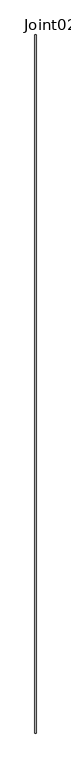
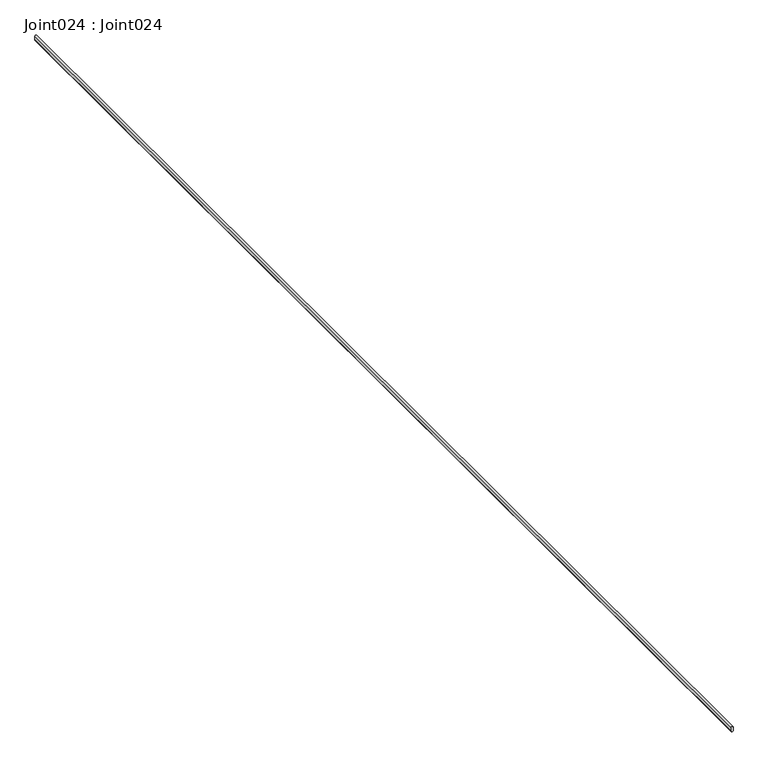
"""IFC4 building model written with IfcOpenShell, lengths in millimetres: proxy geometry, Joint024 : Joint024."""

from ifc_helpers import new_model, si_unit, point, frame, frame_2d, origin, place, context, project, spatial, polyline, circle_curve, trimmed, segment, composite_curve, outline, extrude, source, transform, mapped, element, save


def joint024_joint024_37bc9509(model_context):
    return source(origin(), model_context, "Body", "SweptSolid", [
        extrude(outline(composite_curve([segment(polyline([(42015.0117187, -1061.5223389), (42020.9666748, -1061.5223389)]), True, "CONTINUOUS"), segment(trimmed(circle_curve(frame_2d((42020.9666748, -1063.1082764)), 1.5859375), [point((42020.9666748, -1061.5223389))], [point((42020.9666748, -1064.6942139))], False, "CARTESIAN"), True, "CONTINUOUS"), segment(polyline([(42020.9666748, -1064.6942139), (42015.0117187, -1064.6942139)]), True, "CONTINUOUS"), segment(trimmed(circle_curve(frame_2d((42015.0117187, -1063.1082764)), 1.5859375), [point((42015.0117187, -1064.6942139))], [point((42015.0117187, -1061.5223389))], False, "CARTESIAN"), True, "CONTINUOUS")], self_intersect=False)), frame((0.0, -1052.8906544, 0.0), z_axis=(0.0, 1.0, 0.0), x_axis=(0.0, 0.0, 1.0)), (0.0, 0.0, 1.0), 2000.0),
    ])


if __name__ == "__main__":
    model = new_model("IFC4")
    model_context = context("Model", 3, world=origin())
    ifc_project = project(units=[si_unit("LENGTHUNIT", "METRE", prefix="MILLI")], contexts=[model_context])
    site = spatial("IfcSite", under=ifc_project)
    building = spatial("IfcBuilding", under=site)
    placement = place(None, origin())
    joint024_joint024_shape = joint024_joint024_37bc9509(model_context)
    element("IfcBuildingElementProxy", 1, Name="Joint024 : Joint024", ObjectType="Joint024 : Joint024", at=placement, inside=building, context=model_context, shape_type="MappedRepresentation", body=[
        mapped(joint024_joint024_shape, transform((0.0, 0.0, 0.0), x_axis=(1.0, 0.0, 0.0), y_axis=(0.0, 1.0, 0.0), z_axis=(0.0, 0.0, 1.0))),
    ])
    save(model, "model.ifc")

# Revit data of these elements
# Type "Joint024 : Joint024"
#   NameOverride = "Joint024"
# Element 1 (IfcBuildingElementProxy, "Joint024 : Joint024")
#   Materials on its faces: "SILICON JOINT"
# Materials
#   "SILICON JOINT": class "Unassigned", colour RGB 150 184 127, transparency 0
